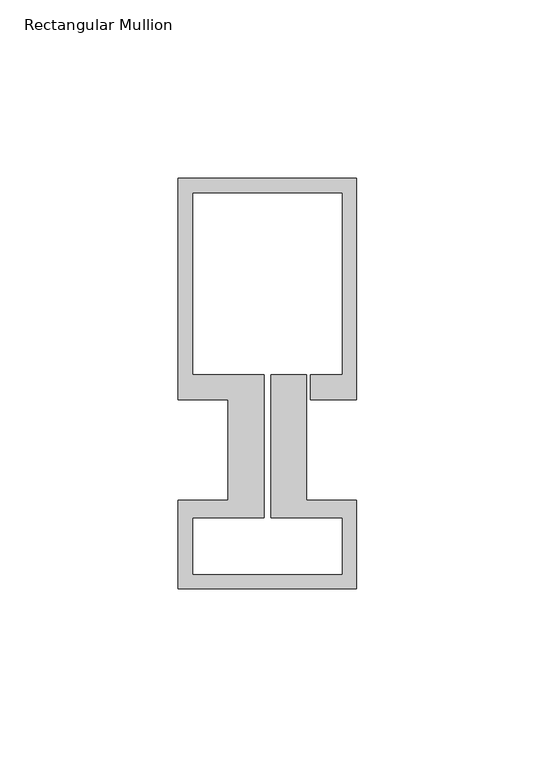
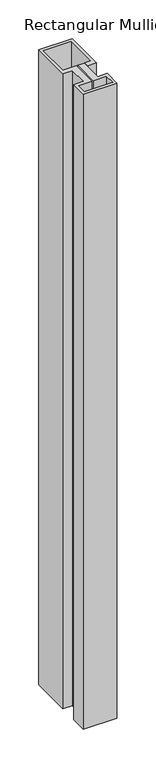
"""IFC4 building model written with IfcOpenShell, lengths in millimetres: member geometry, Rectangular Mullion : Schueco_FWS-50-HI_Tran_CovCap-20mm_Tran-55mm."""

from ifc_helpers import new_model, si_unit, frame, origin, place, context, project, spatial, polyline, outline, extrude, source, transform, mapped, element, save


def rectangular_mullion_3b4738ba(model_context):
    return source(origin(), model_context, "Body", "SweptSolid", [
        extrude(outline(polyline([(-50.0, 90.0), (0.0, 90.0), (0.0, 28.0), (-13.0, 28.0), (-13.0, 35.0), (-4.0, 35.0), (-4.0, 86.0), (-46.0, 86.0), (-46.0, 35.0), (-26.0, 35.0), (-26.0, -5.0), (-46.0, -5.0), (-46.0, -21.0), (-4.0, -21.0), (-4.0, -5.0), (-24.0, -5.0), (-24.0, 35.0), (-14.0, 35.0), (-14.0, -0.1), (0.0, -0.1), (0.0, -25.0), (-50.0, -25.0), (-50.0, -0.1), (-36.0, -0.1), (-36.0, 28.0), (-50.0, 28.0), (-50.0, 90.0)])), frame((0.0, 0.0, -1000.0), z_axis=(0.0, 0.0, 1.0), x_axis=(1.0, 0.0, 0.0)), (0.0, 0.0, 1.0), 1000.0),
    ])


if __name__ == "__main__":
    model = new_model("IFC4")
    model_context = context("Model", 3, world=origin())
    ifc_project = project(units=[si_unit("LENGTHUNIT", "METRE", prefix="MILLI")], contexts=[model_context])
    site = spatial("IfcSite", under=ifc_project)
    building = spatial("IfcBuilding", under=site)
    placement = place(None, origin())
    rectangular_mullion_shape = rectangular_mullion_3b4738ba(model_context)
    element("IfcMember", 1, ObjectType="Rectangular Mullion : Schueco_FWS-50-HI_Tran_CovCap-20mm_Tran-55mm", at=placement, inside=building, context=model_context, shape_type="MappedRepresentation", body=[
        mapped(rectangular_mullion_shape, transform((0.0, 0.0, 0.0), x_axis=(1.0, 0.0, 0.0), y_axis=(0.0, 1.0, 0.0), z_axis=(0.0, 0.0, 1.0))),
    ])
    save(model, "model.ifc")

# Revit data of these elements
# Type "Rectangular Mullion : Schueco_FWS-50-HI_Tran_CovCap-20mm_Tran-55mm"
#   Model = "FWS 50.HI"
#   Manufacturer = "Schueco International KG"
#   Type Comments = "Transom"
#   Schueco thermal insulation standard = "Highly thermally insulated"
#   Burglar resistance = "RC 3"
#   Thermal insulation = "to 0.90 W/(m²K)"
#   built-in parameter 1007322 = 0.377297 (stored number, unit not read)
#   built-in parameter 1007321 = 0.0360892 (stored number, unit not read)
#   built-in parameter 1007320 = 0.0360892 (stored number, unit not read)
# Element 1 (IfcMember, "Rectangular Mullion : Schueco_FWS-50-HI_Tran_CovCap-20mm_Tran-55mm")
#   Materials on its faces: "Alu"
# Materials
#   "Alu": class "Glas", colour RGB 140 140 140, transparency 0
